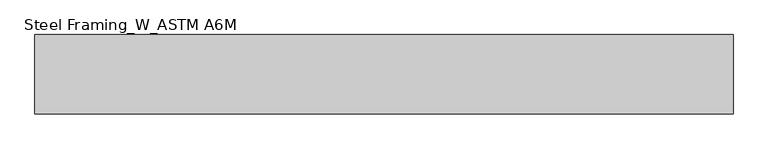
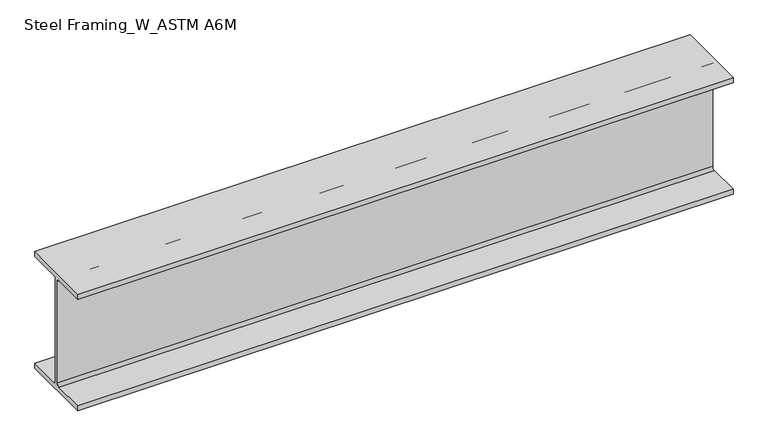
"""IFC4 building model written with IfcOpenShell, lengths in millimetres: beam geometry, Steel Framing_W_ASTM A6M : H_SB_AR_S02_W460x128_B1."""

from ifc_helpers import new_model, si_unit, point, frame, frame_2d, origin, place, context, project, spatial, polyline, circle_curve, trimmed, segment, composite_curve, outline, extrude, source, transform, mapped, element, save


def steel_framing_w_astm_a6m_a62a5a3f(model_context):
    return source(origin(), model_context, "Body", "SweptSolid", [
        extrude(outline(composite_curve([segment(polyline([(141.0, -213.9), (141.0, -233.5), (-141.0, -233.5), (-141.0, -213.9), (-16.2, -213.9)]), True, "CONTINUOUS"), segment(trimmed(circle_curve(frame_2d((-16.2, -203.8)), 10.1), [point((-16.2, -213.9))], [point((-6.1, -203.8))], True, "CARTESIAN"), True, "CONTINUOUS"), segment(polyline([(-6.1, -203.8), (-6.1, 203.8)]), True, "CONTINUOUS"), segment(trimmed(circle_curve(frame_2d((-16.2, 203.8)), 10.1), [point((-6.1, 203.8))], [point((-16.2, 213.9))], True, "CARTESIAN"), True, "CONTINUOUS"), segment(polyline([(-16.2, 213.9), (-141.0, 213.9), (-141.0, 233.5), (141.0, 233.5), (141.0, 213.9), (16.2, 213.9)]), True, "CONTINUOUS"), segment(trimmed(circle_curve(frame_2d((16.2, 203.8)), 10.1), [point((16.2, 213.9))], [point((6.1, 203.8))], True, "CARTESIAN"), True, "CONTINUOUS"), segment(polyline([(6.1, 203.8), (6.1, -203.8)]), True, "CONTINUOUS"), segment(trimmed(circle_curve(frame_2d((16.2, -203.8)), 10.1), [point((6.1, -203.8))], [point((16.2, -213.9))], True, "CARTESIAN"), True, "CONTINUOUS"), segment(polyline([(16.2, -213.9), (141.0, -213.9)]), True, "CONTINUOUS")], self_intersect=False)), frame((-1346.3, 0.0, 0.0), z_axis=(1.0, 0.0, 0.0), x_axis=(0.0, 1.0, 0.0)), (0.0, 0.0, 1.0), 2479.6),
    ])


if __name__ == "__main__":
    model = new_model("IFC4")
    model_context = context("Model", 3, world=origin())
    ifc_project = project(units=[si_unit("LENGTHUNIT", "METRE", prefix="MILLI")], contexts=[model_context])
    site = spatial("IfcSite", under=ifc_project)
    building = spatial("IfcBuilding", under=site)
    placement = place(None, origin())
    steel_framing_w_astm_a6m_shape = steel_framing_w_astm_a6m_a62a5a3f(model_context)
    element("IfcBeam", 1, ObjectType="Steel Framing_W_ASTM A6M : H_SB_AR_S02_W460x128_B1", at=placement, inside=building, context=model_context, shape_type="MappedRepresentation", body=[
        mapped(steel_framing_w_astm_a6m_shape, transform((0.0, 0.0, 0.0), x_axis=(1.0, 0.0, 0.0), y_axis=(0.0, 1.0, 0.0), z_axis=(0.0, 0.0, 1.0))),
    ])
    save(model, "model.ifc")

# Revit data of these elements
# Type "Steel Framing_W_ASTM A6M : H_SB_AR_S02_W460x128_B1"
#   Section Name Key = "W18x86"
#   Width = 28.2 cm
#   Web Thickness = 1.22 cm
#   Web Fillet = 1.01 cm
#   Warping Constant = 3650000.0 cm⁶
#   Torsional Moment of Inertia = 171.00 cm⁴
#   Section Area = 163.0 cm²
#   Plastic Modulus weak axis = 793.0 cm³
#   Plastic Modulus strong axis = 3050.0 cm³
#   Perimeter = 2.02 m²/m
#   Nominal Weight = 128.00 kgf/m
#   Moment of Inertia weak axis = 7280.00 cm⁴
#   Moment of Inertia strong axis = 63700.00 cm⁴
#   Height = 46.7 cm
#   Flange Thickness = 1.96 cm
#   Elastic Modulus weak axis = 518.0 cm³
#   Elastic Modulus strong axis = 2720.0 cm³
#   Centroid Vertical = 23.35 cm
#   Centroid Horizontal = 14.1 cm
#   Length [instance default] = 1500 mm
#   Structural Material [instance default] = Steel, 45-345
#   Bolt Spacing = 0
#   Assembly Code = ""
# Element 1 (IfcBeam, "Steel Framing_W_ASTM A6M : H_SB_AR_S02_W460x128_B1")
#   Materials on its faces: "Steel, 45-345"
# Materials
#   "Steel, 45-345": class "Metal", colour RGB 189 187 185, transparency 0, Description = "Steel 345 MPa", Cost = 0
